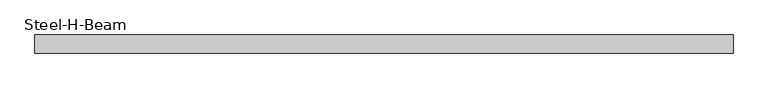
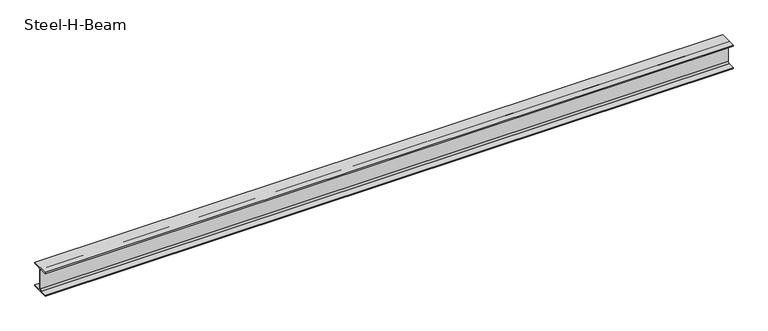
"""IFC4 building model written with IfcOpenShell, lengths in millimetres: beam geometry, Steel-H-Beam : BM121_H-244×175x7x11."""

from ifc_helpers import new_model, si_unit, point, frame, frame_2d, origin, place, context, project, spatial, polyline, circle_curve, trimmed, segment, composite_curve, outline, extrude, source, transform, mapped, element, save


def steel_h_beam_22148b76(model_context):
    return source(origin(), model_context, "Body", "SweptSolid", [
        extrude(outline(composite_curve([segment(polyline([(87.5, -111.0), (87.5, -122.0), (-87.5, -122.0), (-87.5, -111.0), (-19.5, -111.0)]), True, "CONTINUOUS"), segment(trimmed(circle_curve(frame_2d((-19.5, -95.0)), 16.0), [point((-19.5, -111.0))], [point((-3.5, -95.0))], True, "CARTESIAN"), True, "CONTINUOUS"), segment(polyline([(-3.5, -95.0), (-3.5, 95.0)]), True, "CONTINUOUS"), segment(trimmed(circle_curve(frame_2d((-19.5, 95.0)), 16.0), [point((-3.5, 95.0))], [point((-19.5, 111.0))], True, "CARTESIAN"), True, "CONTINUOUS"), segment(polyline([(-19.5, 111.0), (-87.5, 111.0), (-87.5, 122.0), (87.5, 122.0), (87.5, 111.0), (19.5, 111.0)]), True, "CONTINUOUS"), segment(trimmed(circle_curve(frame_2d((19.5, 95.0)), 16.0), [point((19.5, 111.0))], [point((3.5, 95.0))], True, "CARTESIAN"), True, "CONTINUOUS"), segment(polyline([(3.5, 95.0), (3.5, -95.0)]), True, "CONTINUOUS"), segment(trimmed(circle_curve(frame_2d((19.5, -95.0)), 16.0), [point((3.5, -95.0))], [point((19.5, -111.0))], True, "CARTESIAN"), True, "CONTINUOUS"), segment(polyline([(19.5, -111.0), (87.5, -111.0)]), True, "CONTINUOUS")], self_intersect=False)), frame((-3361.8243373, 0.0, 0.0), z_axis=(1.0, 0.0, 0.0), x_axis=(0.0, 1.0, 0.0)), (0.0, 0.0, 1.0), 6724.6),
    ])


if __name__ == "__main__":
    model = new_model("IFC4")
    model_context = context("Model", 3, world=origin())
    ifc_project = project(units=[si_unit("LENGTHUNIT", "METRE", prefix="MILLI")], contexts=[model_context])
    site = spatial("IfcSite", under=ifc_project)
    building = spatial("IfcBuilding", under=site)
    placement = place(None, origin())
    steel_h_beam_shape = steel_h_beam_22148b76(model_context)
    element("IfcBeam", 1, ObjectType="Steel-H-Beam : BM121_H-244×175x7x11", at=placement, inside=building, context=model_context, shape_type="MappedRepresentation", body=[
        mapped(steel_h_beam_shape, transform((0.0, 0.0, 0.0), x_axis=(1.0, 0.0, 0.0), y_axis=(0.0, 1.0, 0.0), z_axis=(0.0, 0.0, 1.0))),
    ])
    save(model, "model.ifc")

# Revit data of these elements
# Type "Steel-H-Beam : BM121_H-244×175x7x11"
#   Surface Area = 1.14653 m²/m
#   Section Area = 56.2375 cm²
#   Mass per Unit Length = 44.1465 kg/m
#   Length [instance default] = 3000 mm
#   B = 175 mm
#   H = 244 mm
#   r = 16 mm
#   tw = 7 mm
#   tf = 11 mm
#   hec_material4 [instance default] = none
#   hec_material3 [instance default] = none
#   hec_material2 [instance default] = none
#   hec_material1 [instance default] = none
#   Structural Material [instance default] = Steel, 45-345
#   Assembly Code = ""
# Element 1 (IfcBeam, "Steel-H-Beam : BM121_H-244×175x7x11")
#   Structural Material = S03AA028-00001_Main Steel Structure Erection Work_Shelter/Building_Medium Steel
#   Materials on its faces: "S03AA028-00001_Main Steel Structure Erection Work_Shelter/Building_Medium Steel"
# Materials
#   "Steel, 45-345": class "Metal", colour RGB 189 187 185, transparency 0, Description = "Steel 345 MPa", Cost = 0
#   "S03AA028-00001_Main Steel Structure Erection Work_Shelter/Building_Medium Steel": class "Metal", colour RGB 120 120 120, transparency 0, Comments = "(90KG/M>Weight≥30KG/M)", Description = "Structural steel 50ksi", W00) Work Master Code = "S03AA028-0001", W01) Work Master_Lv1 = "Main Steel Structure Erection Work", W02) Work Master_Lv2 = "Shelter/Building", W03) Work Master_Spec.1 = "Medium Steel (90KG/M>Weight≥30KG/M)", Cost = 0
